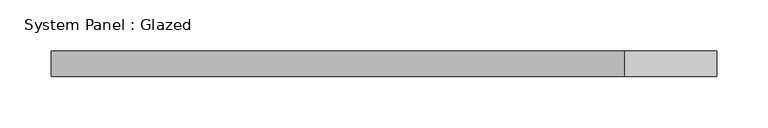
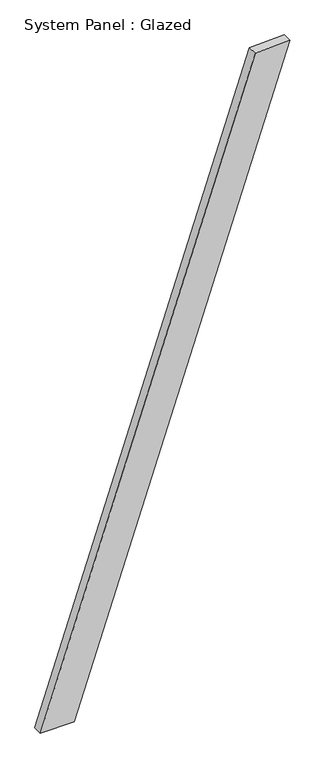
"""IFC4 building model written with IfcOpenShell, lengths in millimetres: plate geometry, System Panel : Glazed."""

from ifc_helpers import new_model, si_unit, frame, origin, place, context, project, spatial, polyline, outline, extrude, source, transform, mapped, element, save


def system_panel_glazed_a4e4dccf(model_context):
    return source(origin(), model_context, "Body", "SweptSolid", [
        extrude(outline(polyline([(0.0, -325.543097), (0.0, -237.614324), (1681.7537152, 325.543097), (1678.0689215, 235.3391836), (0.0, -325.543097)])), frame((0.0, -49.5, 0.0), z_axis=(0.0, 1.0, 0.0), x_axis=(0.0, 0.0, 1.0)), (0.0, 0.0, 1.0), 25.0),
    ])


if __name__ == "__main__":
    model = new_model("IFC4")
    model_context = context("Model", 3, world=origin())
    ifc_project = project(units=[si_unit("LENGTHUNIT", "METRE", prefix="MILLI")], contexts=[model_context])
    site = spatial("IfcSite", under=ifc_project)
    building = spatial("IfcBuilding", under=site)
    placement = place(None, origin())
    system_panel_glazed_shape = system_panel_glazed_a4e4dccf(model_context)
    element("IfcPlate", 1, ObjectType="System Panel : Glazed", at=placement, inside=building, context=model_context, shape_type="MappedRepresentation", body=[
        mapped(system_panel_glazed_shape, transform((0.0, 0.0, 0.0), x_axis=(1.0, 0.0, 0.0), y_axis=(0.0, 1.0, 0.0), z_axis=(0.0, 0.0, 1.0))),
    ])
    save(model, "model.ifc")

# Revit data of these elements
# Element 1 (IfcPlate, "System Panel : Glazed")
#   Materials on its faces: "Glass, Clear Glazing"
# Materials
#   "Glass, Clear Glazing": class "Glass", colour RGB 247 249 248, transparency 0.85, Description = "Clear glazing", Cost = 0
